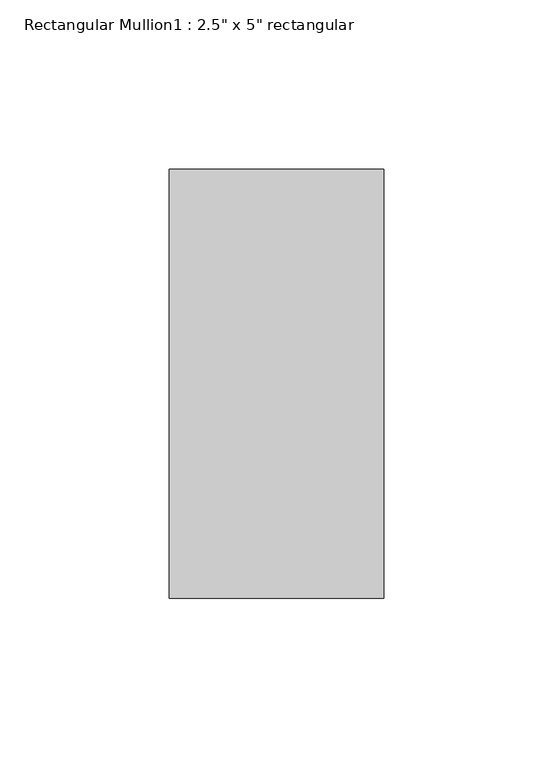
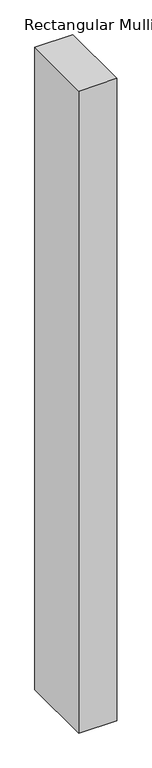
"""IFC4 building model written with IfcOpenShell, lengths in millimetres: member geometry."""

from ifc_helpers import new_model, si_unit, frame, origin, place, context, project, spatial, polyline, outline, extrude, source, transform, mapped, element, save


def member_01a4c065(model_context):
    return source(origin(), model_context, "Body", "SweptSolid", [
        extrude(outline(polyline([(31.75, 63.5), (31.75, -63.5), (-31.75, -63.5), (-31.75, 63.5), (31.75, 63.5)])), frame((0.0, 0.0, -1134.5333334), z_axis=(0.0, 0.0, 1.0), x_axis=(1.0, 0.0, 0.0)), (0.0, 0.0, 1.0), 1134.5333334),
    ])


if __name__ == "__main__":
    model = new_model("IFC4")
    model_context = context("Model", 3, world=origin())
    ifc_project = project(units=[si_unit("LENGTHUNIT", "METRE", prefix="MILLI")], contexts=[model_context])
    site = spatial("IfcSite", under=ifc_project)
    building = spatial("IfcBuilding", under=site)
    placement = place(None, origin())
    member_shape = member_01a4c065(model_context)
    element("IfcMember", 1, ObjectType="Rectangular Mullion1 : 2.5\" x 5\" rectangular", at=placement, inside=building, context=model_context, shape_type="MappedRepresentation", body=[
        mapped(member_shape, transform((0.0, 0.0, 0.0), x_axis=(1.0, 0.0, 0.0), y_axis=(0.0, 1.0, 0.0), z_axis=(0.0, 0.0, 1.0))),
    ])
    save(model, "model.ifc")

# Revit data of these elements
# Type "Rectangular Mullion1 : 2.5\" x 5\" rectangular"
#   built-in parameter 1007304 = 0.416667 (stored number, unit not read)
#   built-in parameter 1007301 = 0.104167 (stored number, unit not read)
#   built-in parameter 1007300 = 0.104167 (stored number, unit not read)
# Element 1 (IfcMember, "Rectangular Mullion1 : 2.5\" x 5\" rectangular")
#   Materials on its faces: "support-frame"
# Materials
#   "support-frame": class "Unassigned", colour RGB 233 233 233, transparency 0, Cost = 0
